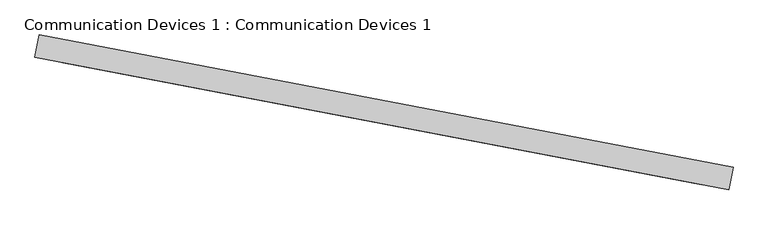
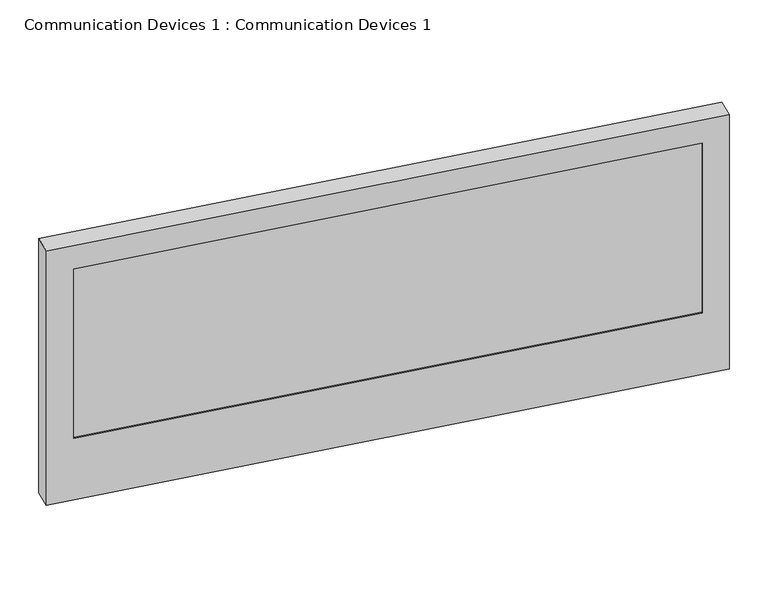
"""IFC4 building model written with IfcOpenShell, lengths in millimetres: proxy geometry, Communication Devices 1 : Communication Devices 1."""

from ifc_helpers import new_model, si_unit, origin, place, context, project, spatial, faceted_brep, source, transform, mapped, element, save


def communication_devices_1_communication_devices_1_7c89eb48(model_context):
    return source(origin(), model_context, "Body", "Brep", [
        faceted_brep([(-9894.8541453, 4429.8973195, 2100.0), (-9924.3709788, 4275.2896983, 2100.0), (-5123.873098, 3358.8051451, 2100.0), (-5094.3562645, 3513.4127663, 2100.0), (-9894.8541453, 4429.8973195, 0.0), (-5094.3562645, 3513.4127663, 0.0), (-5123.873098, 3358.8051451, 0.0), (-9924.3709788, 4275.2896983, 0.0), (-9732.5937318, 4238.676645, 1908.1269566), (-5312.4266701, 3394.8027521, 1908.1269566), (-5312.4266701, 3394.8027521, 508.1269566), (-9732.5937318, 4238.676645, 508.1269566), (-5310.5513948, 3404.6253456, 1908.1269566), (-9730.7184564, 4248.4992385, 1908.1269566), (-9730.7184564, 4248.4992385, 508.1269566), (-5310.5513948, 3404.6253456, 508.1269566)], [[[0, 1, 2, 3]], [[4, 5, 6, 7]], [[1, 0, 4, 7]], [[2, 1, 7, 6], [8, 9, 10, 11]], [[3, 2, 6, 5]], [[0, 3, 5, 4]], [[12, 13, 14, 15]], [[13, 12, 9, 8]], [[14, 13, 8, 11]], [[15, 14, 11, 10]], [[12, 15, 10, 9]]]),
    ])


if __name__ == "__main__":
    model = new_model("IFC4")
    model_context = context("Model", 3, world=origin())
    ifc_project = project(units=[si_unit("LENGTHUNIT", "METRE", prefix="MILLI")], contexts=[model_context])
    site = spatial("IfcSite", under=ifc_project)
    building = spatial("IfcBuilding", under=site)
    placement = place(None, origin())
    communication_devices_1_communication_devices_1_shape = communication_devices_1_communication_devices_1_7c89eb48(model_context)
    element("IfcBuildingElementProxy", 1, Name="Communication Devices 1 : Communication Devices 1", ObjectType="Communication Devices 1 : Communication Devices 1", at=placement, inside=building, context=model_context, shape_type="MappedRepresentation", body=[
        mapped(communication_devices_1_communication_devices_1_shape, transform((0.0, 0.0, 0.0), x_axis=(1.0, 0.0, 0.0), y_axis=(0.0, 1.0, 0.0), z_axis=(0.0, 0.0, 1.0))),
    ])
    save(model, "model.ifc")

# Revit data of these elements
# Type "Communication Devices 1 : Communication Devices 1"
#   COBie.Type.CreatedBy = "design@eagle.com"
#   COBie.Type.CreatedOn = "2016-09-13T05:47:35"
#   COBie.Type.Name = "Communication Devices_Communication Devices 1_Communication Devices 1"
#   COBie.Type.Category = "n/a"
#   COBie.Type.Description = ""
#   COBie.Type.Manufacturer = ""
#   COBie.Type.ModelNumber = ""
#   COBie.Type.ReplacementCost = 0
#   COBie.Type = yes
